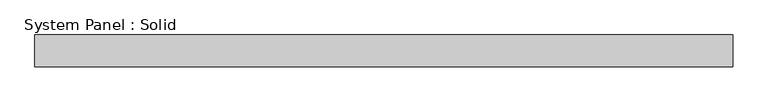
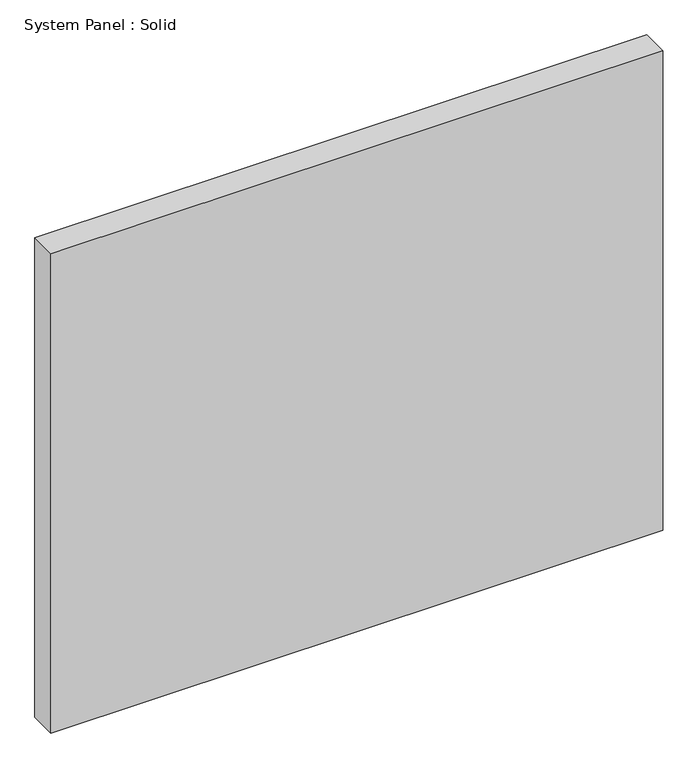
"""IFC4 building model written with IfcOpenShell, lengths in millimetres: plate geometry, System Panel : Solid."""

from ifc_helpers import new_model, si_unit, origin, origin_with_axes, place, context, project, spatial, polyline, outline, extrude, source, transform, mapped, element, save


def system_panel_solid_99af49ff(model_context):
    return source(origin(), model_context, "Body", "SweptSolid", [
        extrude(outline(polyline([(697.4416668, -44.45), (-697.4416668, -44.45), (-697.4416668, 19.05), (697.4416668, 19.05), (697.4416668, -44.45)])), origin_with_axes(), (0.0, 0.0, 1.0), 1155.7),
    ])


if __name__ == "__main__":
    model = new_model("IFC4")
    model_context = context("Model", 3, world=origin())
    ifc_project = project(units=[si_unit("LENGTHUNIT", "METRE", prefix="MILLI")], contexts=[model_context])
    site = spatial("IfcSite", under=ifc_project)
    building = spatial("IfcBuilding", under=site)
    placement = place(None, origin())
    system_panel_solid_shape = system_panel_solid_99af49ff(model_context)
    element("IfcPlate", 1, ObjectType="System Panel : Solid", at=placement, inside=building, context=model_context, shape_type="MappedRepresentation", body=[
        mapped(system_panel_solid_shape, transform((0.0, 0.0, 0.0), x_axis=(1.0, 0.0, 0.0), y_axis=(0.0, 1.0, 0.0), z_axis=(0.0, 0.0, 1.0))),
    ])
    save(model, "model.ifc")

# Revit data of these elements
# Type "System Panel : Solid"
#   Construction Type Id = "MDOOR"
#   Analytic Construction = "Metal"
#   Visual Light Transmittance = 0
#   Solar Heat Gain Coefficient = 0
#   Heat Transfer Coefficient (U) = 0.651978 BTU/(h·ft²·°F)
#   Define Thermal Properties by = 1
# Element 1 (IfcPlate, "System Panel : Solid")
#   Materials on its faces: "Default"
# Materials
#   "Default": class "Miscellaneous", colour RGB 127 127 127, transparency 0, Cost = 0
